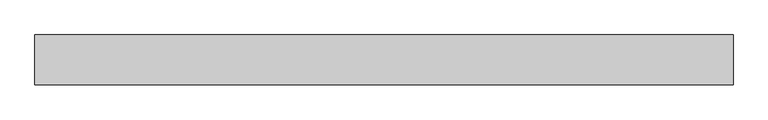
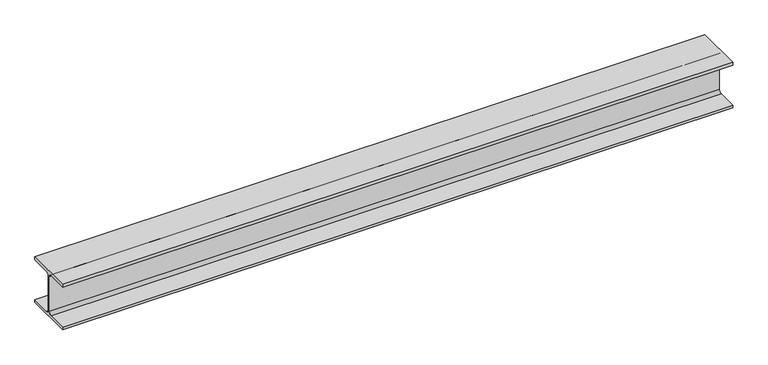
"""IFC4 building model written with IfcOpenShell, lengths in millimetres: beam geometry, 0912_Steel Framing_H-KSD3502 : H_SB_ASB_H-200x200x8x12."""

from ifc_helpers import new_model, si_unit, point, frame, frame_2d, origin, place, context, project, spatial, polyline, circle_curve, trimmed, segment, composite_curve, outline, extrude, source, transform, mapped, element, save


def beam_7a9ba89b(model_context):
    return source(origin(), model_context, "Body", "SweptSolid", [
        extrude(outline(composite_curve([segment(polyline([(100.0, -88.0), (100.0, -100.0), (-100.0, -100.0), (-100.0, -88.0), (-17.0, -88.0)]), True, "CONTINUOUS"), segment(trimmed(circle_curve(frame_2d((-17.0, -75.0)), 13.0), [point((-17.0, -88.0))], [point((-4.0, -75.0))], True, "CARTESIAN"), True, "CONTINUOUS"), segment(polyline([(-4.0, -75.0), (-4.0, 75.0)]), True, "CONTINUOUS"), segment(trimmed(circle_curve(frame_2d((-17.0, 75.0)), 13.0), [point((-4.0, 75.0))], [point((-17.0, 88.0))], True, "CARTESIAN"), True, "CONTINUOUS"), segment(polyline([(-17.0, 88.0), (-100.0, 88.0), (-100.0, 100.0), (100.0, 100.0), (100.0, 88.0), (17.0, 88.0)]), True, "CONTINUOUS"), segment(trimmed(circle_curve(frame_2d((17.0, 75.0)), 13.0), [point((17.0, 88.0))], [point((4.0, 75.0))], True, "CARTESIAN"), True, "CONTINUOUS"), segment(polyline([(4.0, 75.0), (4.0, -75.0)]), True, "CONTINUOUS"), segment(trimmed(circle_curve(frame_2d((17.0, -75.0)), 13.0), [point((4.0, -75.0))], [point((17.0, -88.0))], True, "CARTESIAN"), True, "CONTINUOUS"), segment(polyline([(17.0, -88.0), (100.0, -88.0)]), True, "CONTINUOUS")], self_intersect=False)), frame((-1363.9291779, 0.0, 0.0), z_axis=(1.0, 0.0, 0.0), x_axis=(0.0, 1.0, 0.0)), (0.0, 0.0, 1.0), 2789.3536853),
    ])


if __name__ == "__main__":
    model = new_model("IFC4")
    model_context = context("Model", 3, world=origin())
    ifc_project = project(units=[si_unit("LENGTHUNIT", "METRE", prefix="MILLI")], contexts=[model_context])
    site = spatial("IfcSite", under=ifc_project)
    building = spatial("IfcBuilding", under=site)
    placement = place(None, origin())
    beam_shape = beam_7a9ba89b(model_context)
    element("IfcBeam", 1, ObjectType="0912_Steel Framing_H-KSD3502 : H_SB_ASB_H-200x200x8x12", at=placement, inside=building, context=model_context, shape_type="MappedRepresentation", body=[
        mapped(beam_shape, transform((0.0, 0.0, 0.0), x_axis=(1.0, 0.0, 0.0), y_axis=(0.0, 1.0, 0.0), z_axis=(0.0, 0.0, 1.0))),
    ])
    save(model, "model.ifc")

# Revit data of these elements
# Type "0912_Steel Framing_H-KSD3502 : H_SB_ASB_H-200x200x8x12"
#   H_WM Code_1 = "S01AA002-00001 | Main Steel Structure Fabrication Work | Shelter/Building | Medium Steel - Standard (90KG/M>Weight≥30KG/M) | Material: (   )"
#   H_WM Code_2 = "S03AA028-00001 | Main Steel Structure Erection Work | Shelter/Building | Medium Steel (90KG/M>Weight≥30KG/M) | Material: (   )"
#   H_WM Code_3 = "S01AA010-00001 | Main Steel Structure Fabrication Work | Shelter/Building | Steel Painting/Coating | for Non-Fireproofed Steel Surface, Surface Preparation, Primer, Second & Final Coat | Material: (   )"
#   H_Q'ty Cal Type Tag = "SB-Q2"
#   Width = 20.0 cm
#   Web Thickness = 0.8 cm
#   Web Fillet = 1.3 cm
#   Warping Constant = 141000.0 cm⁶
#   W = 0
#   Torsional Moment of Inertia = 26.2485 cm⁴
#   Section Area = 63.53 cm²
#   Plastic Modulus weak axis = 244.0 cm³
#   Plastic Modulus strong axis = 525.0 cm³
#   Perimeter = 1.16 m²/m
#   Nominal Weight = 49.90 kgf/m
#   Moment of Inertia weak axis = 1600.00 cm⁴
#   Moment of Inertia strong axis = 4720.00 cm⁴
#   Height = 20.0 cm
#   Flange Thickness = 1.2 cm
#   Elastic Modulus weak axis = 160.0 cm³
#   Elastic Modulus strong axis = 472.0 cm³
#   Centroid Vertical = 10.0 cm
#   Centroid Horizontal = 10.0 cm
#   Ix = 47200000
#   Length [instance default] = 1.5240 m
#   Zx = 525000
#   b = 0.2000 m
#   h = 0.2000 m
#   r = 0.0130 m
#   s = 0.0080 m
#   t = 0.0120 m
#   A = 0.006353 m²
#   Structural Material [instance default] = Steel, 45-345
#   Assembly Code = ""
# Element 1 (IfcBeam, "0912_Steel Framing_H-KSD3502 : H_SB_ASB_H-200x200x8x12")
#   Structural Material = none
# Materials
#   "Steel, 45-345": class "Metal", colour RGB 189 187 185, transparency 0, Description = "Steel 345 MPa", Cost = 0
